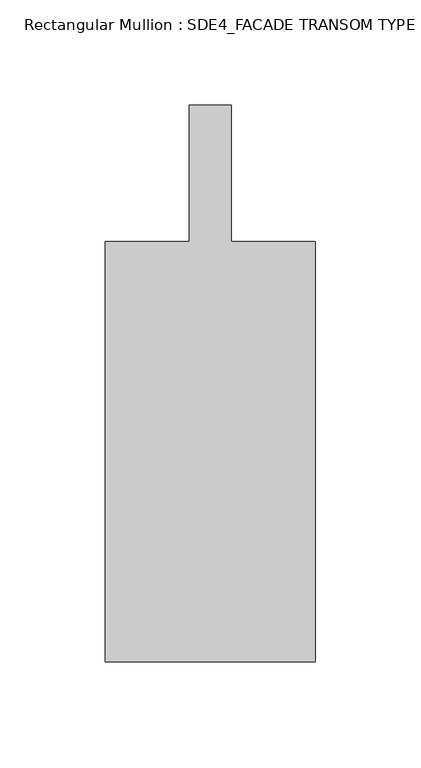
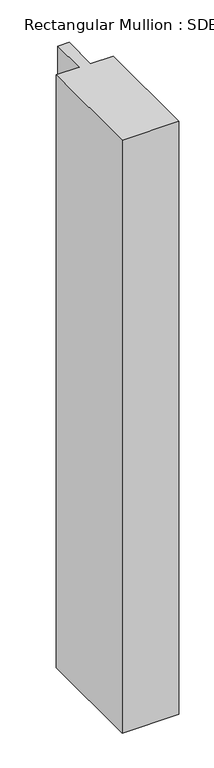
"""IFC4 building model written with IfcOpenShell, lengths in millimetres: member geometry, Rectangular Mullion : SDE4_FACADE TRANSOM TYPE 2."""

from ifc_helpers import new_model, si_unit, frame, origin, place, context, project, spatial, polyline, outline, extrude, source, transform, mapped, element, save


def rectangular_mullion_sde4_facade_transom_type_2_582a2491(model_context):
    return source(origin(), model_context, "Body", "SweptSolid", [
        extrude(outline(polyline([(50.0, -132.5), (-50.0, -132.5), (-50.0, 67.5), (-10.0, 67.5), (-10.0, 132.5), (10.0, 132.5), (10.0, 67.5), (50.0, 67.5), (50.0, -132.5)])), frame((0.0, 0.0, -1100.9999999), z_axis=(0.0, 0.0, 1.0), x_axis=(1.0, 0.0, 0.0)), (0.0, 0.0, 1.0), 1100.9999999),
    ])


if __name__ == "__main__":
    model = new_model("IFC4")
    model_context = context("Model", 3, world=origin())
    ifc_project = project(units=[si_unit("LENGTHUNIT", "METRE", prefix="MILLI")], contexts=[model_context])
    site = spatial("IfcSite", under=ifc_project)
    building = spatial("IfcBuilding", under=site)
    placement = place(None, origin())
    rectangular_mullion_sde4_facade_transom_type_2_shape = rectangular_mullion_sde4_facade_transom_type_2_582a2491(model_context)
    element("IfcMember", 1, ObjectType="Rectangular Mullion : SDE4_FACADE TRANSOM TYPE 2", at=placement, inside=building, context=model_context, shape_type="MappedRepresentation", body=[
        mapped(rectangular_mullion_sde4_facade_transom_type_2_shape, transform((0.0, 0.0, 0.0), x_axis=(1.0, 0.0, 0.0), y_axis=(0.0, 1.0, 0.0), z_axis=(0.0, 0.0, 1.0))),
    ])
    save(model, "model.ifc")

# Revit data of these elements
# Type "Rectangular Mullion : SDE4_FACADE TRANSOM TYPE 2"
#   built-in parameter 1007322 = 0.869423 (stored number, unit not read)
#   built-in parameter 1007321 = 0.164042 (stored number, unit not read)
#   built-in parameter 1007320 = 0.164042 (stored number, unit not read)
